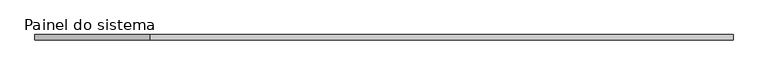
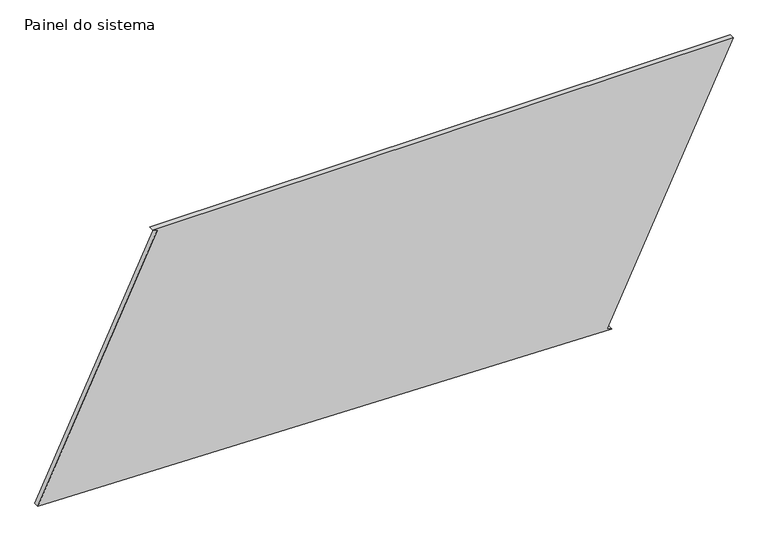
"""IFC4 building model written with IfcOpenShell, lengths in millimetres: plate geometry, Painel do sistema : Envidraçado."""

from ifc_helpers import new_model, si_unit, frame, origin, place, context, project, spatial, polyline, outline, extrude, source, transform, mapped, element, save


def painel_do_sistema_7592c6a3(model_context):
    return source(origin(), model_context, "Body", "SweptSolid", [
        extrude(outline(polyline([(0.0, 1101.0616884), (10.7698497, 1078.5004309), (1292.2724805, 1690.2389697), (1292.2724805, -1132.7740453), (1281.5026308, -1110.2127879), (66.4327426, -1690.2389697), (0.0, 1101.0616884)])), frame((0.0, 24.5, 0.0), z_axis=(0.0, 1.0, 0.0), x_axis=(0.0, 0.0, 1.0)), (0.0, 0.0, 1.0), 25.0),
    ])


if __name__ == "__main__":
    model = new_model("IFC4")
    model_context = context("Model", 3, world=origin())
    ifc_project = project(units=[si_unit("LENGTHUNIT", "METRE", prefix="MILLI")], contexts=[model_context])
    site = spatial("IfcSite", under=ifc_project)
    building = spatial("IfcBuilding", under=site)
    placement = place(None, origin())
    painel_do_sistema_shape = painel_do_sistema_7592c6a3(model_context)
    element("IfcPlate", 1, ObjectType="Painel do sistema : Envidraçado", at=placement, inside=building, context=model_context, shape_type="MappedRepresentation", body=[
        mapped(painel_do_sistema_shape, transform((0.0, 0.0, 0.0), x_axis=(1.0, 0.0, 0.0), y_axis=(0.0, 1.0, 0.0), z_axis=(0.0, 0.0, 1.0))),
    ])
    save(model, "model.ifc")

# Revit data of these elements
# Type "Painel do sistema : Envidraçado"
#   Construction Type Id = "GSP4R"
#   Analytic Construction = "Vidraça única Pilkington 1/8 pol"
#   Visual Light Transmittance = 0.9
#   Solar Heat Gain Coefficient = 0.86
#   Heat Transfer Coefficient (U) = 6.7069 W/(m²·K)
# Element 1 (IfcPlate, "Painel do sistema : Envidraçado")
#   Materials on its faces: "Vidro"
# Materials
#   "Vidro": class "Vidro", colour RGB 0 128 192, transparency 0.9, Description = "Vidro de sílica", Cost = 0
